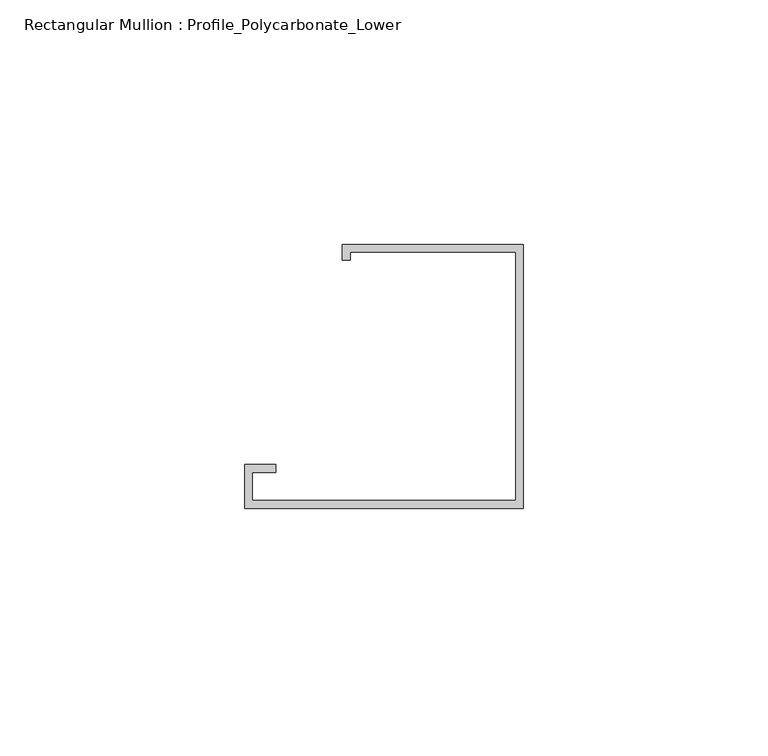
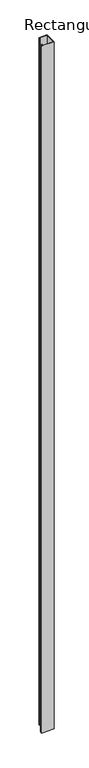
"""IFC4 building model written with IfcOpenShell, lengths in millimetres: member geometry, Rectangular Mullion : Profile_Polycarbonate_Lower."""

from ifc_helpers import new_model, si_unit, frame, origin, place, context, project, spatial, polyline, outline, extrude, source, transform, mapped, element, save


def rectangular_mullion_profile_polycarbonate_lower_12ac12bd(model_context):
    return source(origin(), model_context, "Body", "SweptSolid", [
        extrude(outline(polyline([(0.0, -28.984575), (-56.9976, -28.984575), (-56.9976, -19.992975), (-50.6476, -19.992975), (-50.6476, -21.580475), (-55.4101, -21.580475), (-55.4101, -27.397075), (-1.5875, -27.397075), (-1.5875, 23.428325), (-35.3949, 23.428325), (-35.3949, 21.840825), (-36.9824, 21.840825), (-36.9824, 25.015825), (0.0, 25.015825), (0.0, -28.984575)])), frame((0.0, 0.0, -3288.9773946), z_axis=(0.0, 0.0, 1.0), x_axis=(1.0, 0.0, 0.0)), (0.0, 0.0, 1.0), 3288.9773946),
    ])


if __name__ == "__main__":
    model = new_model("IFC4")
    model_context = context("Model", 3, world=origin())
    ifc_project = project(units=[si_unit("LENGTHUNIT", "METRE", prefix="MILLI")], contexts=[model_context])
    site = spatial("IfcSite", under=ifc_project)
    building = spatial("IfcBuilding", under=site)
    placement = place(None, origin())
    rectangular_mullion_profile_polycarbonate_lower_shape = rectangular_mullion_profile_polycarbonate_lower_12ac12bd(model_context)
    element("IfcMember", 1, ObjectType="Rectangular Mullion : Profile_Polycarbonate_Lower", at=placement, inside=building, context=model_context, shape_type="MappedRepresentation", body=[
        mapped(rectangular_mullion_profile_polycarbonate_lower_shape, transform((0.0, 0.0, 0.0), x_axis=(1.0, 0.0, 0.0), y_axis=(0.0, 1.0, 0.0), z_axis=(0.0, 0.0, 1.0))),
    ])
    save(model, "model.ifc")

# Revit data of these elements
# Type "Rectangular Mullion : Profile_Polycarbonate_Lower"
#   built-in parameter 1007322 = 0.177167 (stored number, unit not read)
#   built-in parameter 1007321 = 0 (stored number, unit not read)
#   built-in parameter 1007320 = 0.00520833 (stored number, unit not read)
